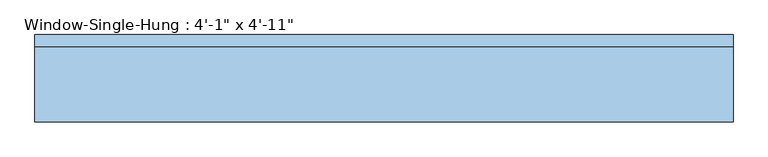
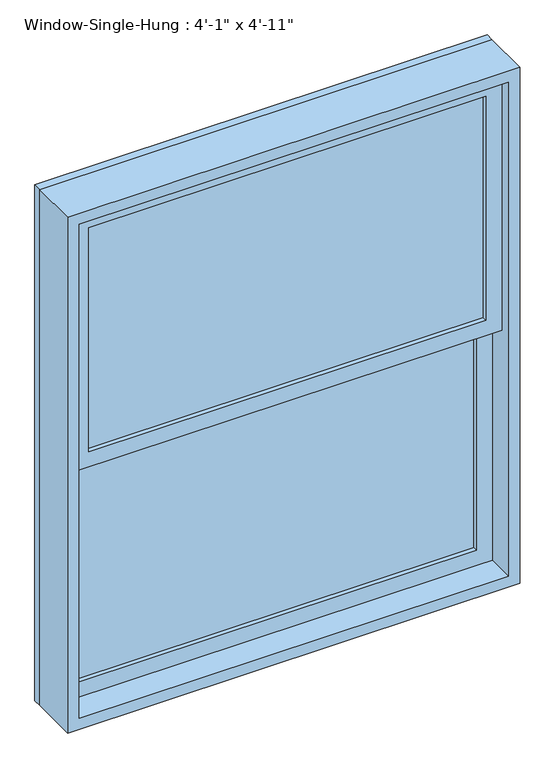
"""IFC4 building model written with IfcOpenShell, lengths in millimetres: window geometry."""

from ifc_helpers import new_model, si_unit, frame, origin, place, context, project, spatial, polyline, outline, extrude, source, transform, mapped, element, save


def window_e1e3fa88(model_context):
    return source(origin(), model_context, "Body", "SweptSolid", [
        extrude(outline(polyline([(546.1, 1.5875), (-546.1, 1.5875), (-546.1, 7.9375), (546.1, 7.9375), (546.1, 1.5875)])), frame((0.0, 0.0, 990.6), z_axis=(0.0, 0.0, 1.0), x_axis=(1.0, 0.0, 0.0)), (0.0, 0.0, 1.0), 650.875),
        extrude(outline(polyline([(-546.1, 14.2875), (-546.1, 20.6375), (546.1, 20.6375), (546.1, 14.2875), (-546.1, 14.2875)])), frame((0.0, 0.0, 990.6), z_axis=(0.0, 0.0, 1.0), x_axis=(1.0, 0.0, 0.0)), (0.0, 0.0, 1.0), 650.875),
        extrude(outline(polyline([(546.1, -42.8625), (-546.1, -42.8625), (-546.1, -36.5125), (546.1, -36.5125), (546.1, -42.8625)])), frame((0.0, 0.0, 1685.925), z_axis=(0.0, 0.0, 1.0), x_axis=(1.0, 0.0, 0.0)), (0.0, 0.0, 1.0), 650.875),
        extrude(outline(polyline([(-546.1, -30.1625), (-546.1, -23.8125), (546.1, -23.8125), (546.1, -30.1625), (-546.1, -30.1625)])), frame((0.0, 0.0, 1685.925), z_axis=(0.0, 0.0, 1.0), x_axis=(1.0, 0.0, 0.0)), (0.0, 0.0, 1.0), 650.875),
        extrude(outline(polyline([(1685.925, 590.55), (1685.925, -590.55), (946.15, -590.55), (946.15, 590.55), (1685.925, 590.55)]), holes=[polyline([(1641.475, -546.1), (1641.475, 546.1), (990.6, 546.1), (990.6, -546.1), (1641.475, -546.1)])]), frame((0.0, -11.1125, 0.0), z_axis=(0.0, 1.0, 0.0), x_axis=(0.0, 0.0, 1.0)), (0.0, 0.0, 1.0), 44.45),
        extrude(outline(polyline([(2381.25, 590.55), (2381.25, -590.55), (1641.475, -590.55), (1641.475, 590.55), (2381.25, 590.55)]), holes=[polyline([(2336.8, -546.1), (2336.8, 546.1), (1685.925, 546.1), (1685.925, -546.1), (2336.8, -546.1)])]), frame((0.0, -55.5625, 0.0), z_axis=(0.0, 1.0, 0.0), x_axis=(0.0, 0.0, 1.0)), (0.0, 0.0, 1.0), 44.45),
        extrude(outline(polyline([(2413.0, 622.3), (2413.0, -622.3), (914.4, -622.3), (914.4, 622.3), (2413.0, 622.3)]), holes=[polyline([(2381.25, -590.55), (2381.25, 590.55), (946.15, 590.55), (946.15, -590.55), (2381.25, -590.55)])]), frame((0.0, -87.3125, 0.0), z_axis=(0.0, 1.0, 0.0), x_axis=(0.0, 0.0, 1.0)), (0.0, 0.0, 1.0), 133.35),
        extrude(outline(polyline([(2413.0, 622.3), (2413.0, -622.3), (914.4, -622.3), (914.4, 622.3), (2413.0, 622.3)]), holes=[polyline([(2393.95, 603.25), (933.45, 603.25), (933.45, -603.25), (2393.95, -603.25), (2393.95, 603.25)])]), frame((0.0, 46.0375, 0.0), z_axis=(0.0, 1.0, 0.0), x_axis=(0.0, 0.0, 1.0)), (0.0, 0.0, 1.0), 22.225),
    ])


if __name__ == "__main__":
    model = new_model("IFC4")
    model_context = context("Model", 3, world=origin())
    ifc_project = project(units=[si_unit("LENGTHUNIT", "METRE", prefix="MILLI")], contexts=[model_context])
    site = spatial("IfcSite", under=ifc_project)
    building = spatial("IfcBuilding", under=site)
    placement = place(None, origin())
    window_shape = window_e1e3fa88(model_context)
    element("IfcWindow", 1, ObjectType="Window-Single-Hung : 4'-1\" x 4'-11\"", at=placement, inside=building, context=model_context, shape_type="MappedRepresentation", body=[
        mapped(window_shape, transform((0.0, 0.0, 0.0), x_axis=(1.0, 0.0, 0.0), y_axis=(0.0, 1.0, 0.0), z_axis=(0.0, 0.0, 1.0))),
    ])
    save(model, "model.ifc")

# Revit data of these elements
# Type "Window-Single-Hung : 4'-1\" x 4'-11\""
#   Type Mark = "20"
#   Fire Rating = "0.5h"
#   Construction Type Id = "DG-DR"
#   Assembly Code = "B2020100"
#   Analytic Construction = "Double glazing - domestic"
#   Wall Thickness [instance default] = 0' - 6"
#   Window Inset [instance default] = 0' - 0"
#   Visual Light Transmittance = 0.81
#   Thermal Resistance (R) = 0.319569 (m²·K)/W
#   Solar Heat Gain Coefficient = 0.76
#   Muntin Width = 3' - 7"
#   Muntin Height = 2' - 1 5/8"
#   Interior Wall Closure [instance default] = 0' - 1 1/2"
#   Rough Width = 4' - 1 1/2"
#   Rough Height = 4' - 11 1/2"
#   Frame Extension [instance default] = 0' - 1 1/4"
#   Exterior Wall Closure [instance default] = 0' - 0 1/2"
#   Extension Jamb [instance default] = 0' - 1 1/2"
#   Heat Transfer Coefficient (U) = 3.12929 W/(m²·K)
#   Height = 4' - 11"
#   Width = 4' - 1"
#   Top Muntin Visibility = yes
#   Indicator Visibility [instance default] = yes
#   Extension Jamb Visibility [instance default] = yes
#   Interior Trim Visibility [instance default] = yes
#   Exterior Trim Visibility [instance default] = yes
#   Bottom Muntin Visibility = yes
#   Muntin Pattern = Muntin Pattern_2x2 : Muntin Pattern_2x2
#   Interior Trim Material = Wood - Stained
#   Interior Trim = Trim-Window-Interior-Flat : Picture Frame
#   Exterior Trim Material = Clad - White
#   Exterior Trim = Trim-Window-Exterior-Flat : with Sill
#   Glass Panel Material = Glass
#   Exterior Frame Material = Clad - White
#   Interior Frame Material = Wood - Stained
#   Wall Closure = (empty or 0)
# Element 1 (IfcWindow, "Window-Single-Hung : 4'-1\" x 4'-11\"")
#   Wall Thickness = 0' - 5 3/8"
#   Extension Jamb = 0' - 0 7/8"
#   Materials on its faces: "Wood - Stained", "Glass", "Clad - White"
# Materials
#   "Wood - Stained": class "Wood", colour RGB 224 178 126, transparency 0, Cost = 0
#   "Clad - White": class "Wood", colour RGB 242 242 238, transparency 0, Cost = 0
#   "Glass": class "Glass", colour RGB 0 128 192, transparency 0.75, Description = "Soda Lime Glass", Cost = 0
